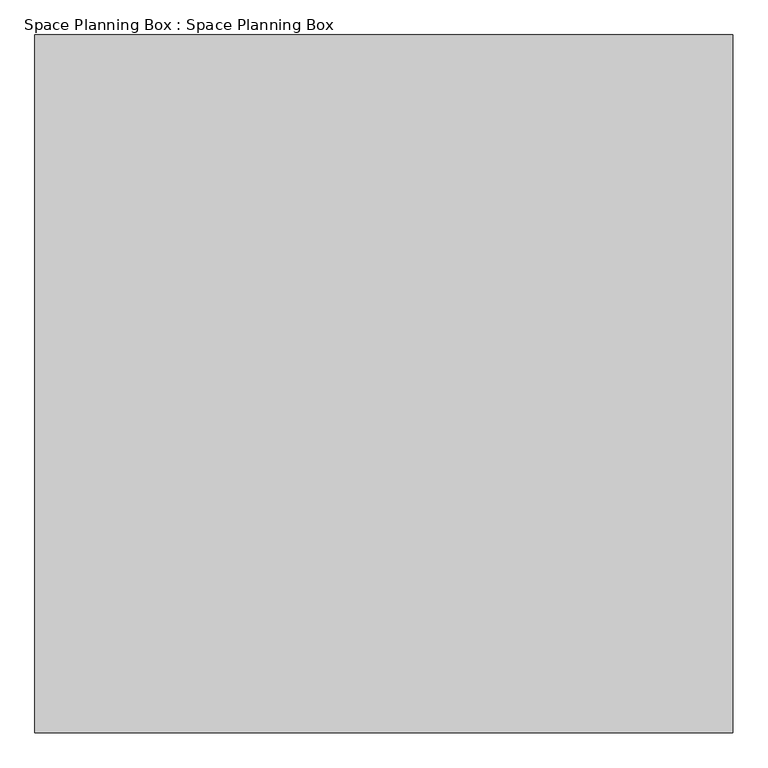
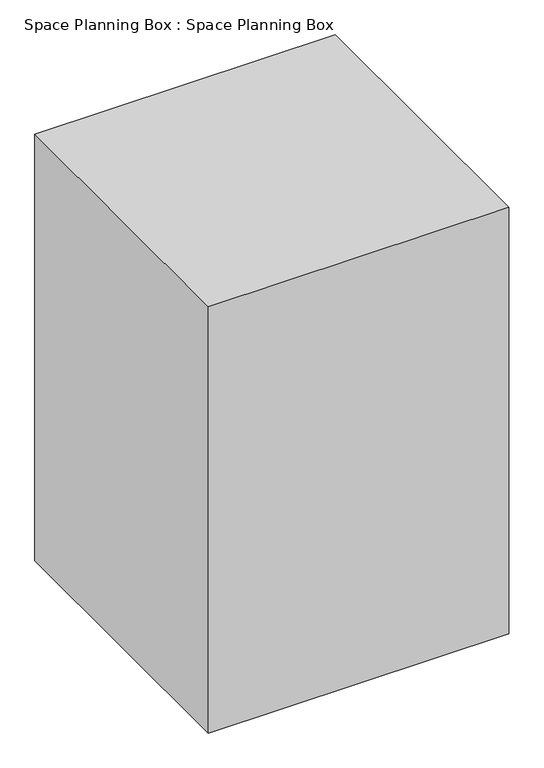
"""IFC4 building model written with IfcOpenShell, lengths in millimetres: proxy geometry, Space Planning Box : Space Planning Box."""

from ifc_helpers import new_model, si_unit, origin, origin_with_axes, place, context, project, spatial, polyline, outline, extrude, source, transform, mapped, element, save


def space_planning_box_space_planning_box_7bff30ad(model_context):
    return source(origin(), model_context, "Body", "SweptSolid", [
        extrude(outline(polyline([(2000.0, 2000.0), (2000.0, -2000.0), (-2000.0, -2000.0), (-2000.0, 2000.0), (2000.0, 2000.0)])), origin_with_axes(), (0.0, 0.0, 1.0), 6000.0),
    ])


if __name__ == "__main__":
    model = new_model("IFC4")
    model_context = context("Model", 3, world=origin())
    ifc_project = project(units=[si_unit("LENGTHUNIT", "METRE", prefix="MILLI")], contexts=[model_context])
    site = spatial("IfcSite", under=ifc_project)
    building = spatial("IfcBuilding", under=site)
    placement = place(None, origin())
    space_planning_box_space_planning_box_shape = space_planning_box_space_planning_box_7bff30ad(model_context)
    element("IfcBuildingElementProxy", 1, Name="Space Planning Box : Space Planning Box", ObjectType="Space Planning Box : Space Planning Box", at=placement, inside=building, context=model_context, shape_type="MappedRepresentation", body=[
        mapped(space_planning_box_space_planning_box_shape, transform((0.0, 0.0, 0.0), x_axis=(1.0, 0.0, 0.0), y_axis=(0.0, 1.0, 0.0), z_axis=(0.0, 0.0, 1.0))),
    ])
    save(model, "model.ifc")

# Revit data of these elements
# Type "Space Planning Box : Space Planning Box"
#   Type Comments = "..."
#   Room Name [instance default] = "?"
#   Assembly Code = "..."
#   Width [instance default] = 1524 mm
#   Program Area [instance default] = 0 m²
#   Length [instance default] = 1524 mm
#   Height [instance default] = 1524 mm
#   Area [instance default] = 2.32258 m²
#   Fill Color [instance default] = Cyan
#   Default Elevation = 0
# Element 1 (IfcBuildingElementProxy, "Space Planning Box : Space Planning Box")
#   Room Name = "Toilet (F)"
#   Width = 4000 mm
#   Program Area = 72 m²
#   Length = 4000 mm
#   Height = 6000 mm
#   Area = 16 m²
#   Fill Color = Lavender
#   Materials on its faces: "Lavender"
# Materials
#   "Cyan": class "Generic", colour RGB 0 255 255, transparency 0.2, Cost = 0
#   "Lavender": class "Generic", colour RGB 186 85 211, transparency 0.2, Cost = 0
